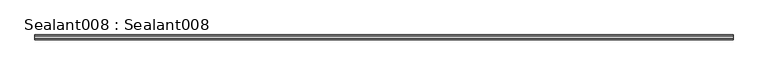
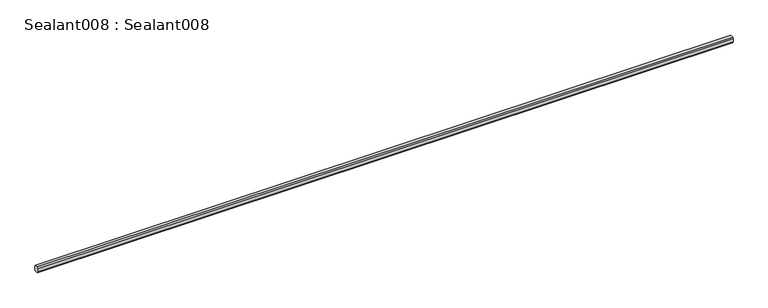
"""IFC4 building model written with IfcOpenShell, lengths in millimetres: proxy geometry, Sealant008 : Sealant008."""

from ifc_helpers import new_model, si_unit, frame, origin, place, context, project, spatial, polyline, outline, extrude, source, transform, mapped, element, save


def sealant008_sealant008_870e320b(model_context):
    return source(origin(), model_context, "Body", "SweptSolid", [
        extrude(outline(polyline([(9625.6284211, 37626.0840792), (9628.3313468, 37629.5137666), (9637.6015625, 37629.5137666), (9639.8066406, 37625.4707979), (9639.8066406, 37617.1426729), (9637.1113281, 37612.6075166), (9628.0862296, 37612.6075166), (9625.6284211, 37617.1138617), (9625.6284211, 37626.0840792)])), frame((-9232.0719278, 0.0, 0.0), z_axis=(1.0, 0.0, 0.0), x_axis=(0.0, 1.0, 0.0)), (0.0, 0.0, 1.0), 1999.85),
    ])


if __name__ == "__main__":
    model = new_model("IFC4")
    model_context = context("Model", 3, world=origin())
    ifc_project = project(units=[si_unit("LENGTHUNIT", "METRE", prefix="MILLI")], contexts=[model_context])
    site = spatial("IfcSite", under=ifc_project)
    building = spatial("IfcBuilding", under=site)
    placement = place(None, origin())
    sealant008_sealant008_shape = sealant008_sealant008_870e320b(model_context)
    element("IfcBuildingElementProxy", 1, Name="Sealant008 : Sealant008", ObjectType="Sealant008 : Sealant008", at=placement, inside=building, context=model_context, shape_type="MappedRepresentation", body=[
        mapped(sealant008_sealant008_shape, transform((0.0, 0.0, 0.0), x_axis=(1.0, 0.0, 0.0), y_axis=(0.0, 1.0, 0.0), z_axis=(0.0, 0.0, 1.0))),
    ])
    save(model, "model.ifc")

# Revit data of these elements
# Type "Sealant008 : Sealant008"
#   NameOverride = "Sealant008"
# Element 1 (IfcBuildingElementProxy, "Sealant008 : Sealant008")
#   Materials on its faces: "BACKER ROD"
# Materials
#   "BACKER ROD": class "Unassigned", colour RGB 214 176 139, transparency 0, Cost = 0
